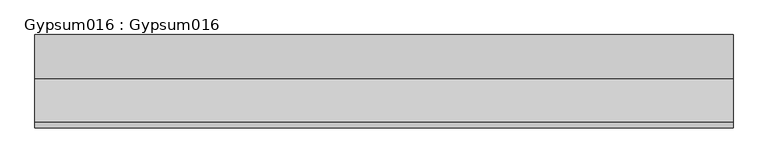
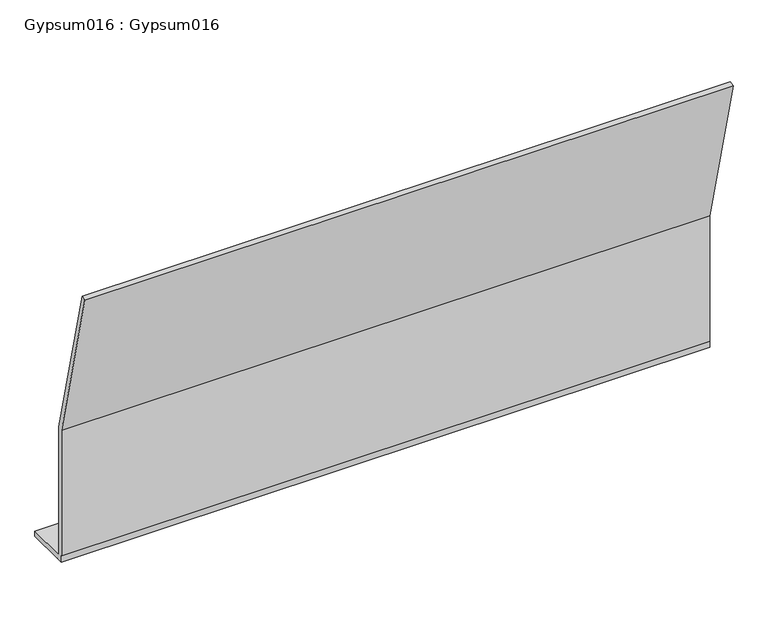
"""IFC4 building model written with IfcOpenShell, lengths in millimetres: proxy geometry, Gypsum016 : Gypsum016."""

from ifc_helpers import new_model, si_unit, frame, origin, place, context, project, spatial, polyline, outline, extrude, source, transform, mapped, element, save


def gypsum016_gypsum016_12ec1e8b(model_context):
    return source(origin(), model_context, "Body", "SweptSolid", [
        extrude(outline(polyline([(10278.0250834, 42906.696), (10404.7574604, 42906.696), (10404.7574604, 42890.821), (10284.5832673, 42890.821), (10284.5832673, 42892.101), (10263.4300834, 42892.101), (10263.4300834, 42913.2541839), (10262.1500834, 42913.2541839), (10262.1500834, 43322.8477886), (10137.3940009, 43821.8721184), (10152.7950131, 43825.7223714), (10278.0250834, 43324.8020904), (10278.0250834, 42906.696)])), frame((3694.2883192, 0.0, 0.0), z_axis=(1.0, 0.0, 0.0), x_axis=(0.0, 1.0, 0.0)), (0.0, 0.0, 1.0), 2000.0),
    ])


if __name__ == "__main__":
    model = new_model("IFC4")
    model_context = context("Model", 3, world=origin())
    ifc_project = project(units=[si_unit("LENGTHUNIT", "METRE", prefix="MILLI")], contexts=[model_context])
    site = spatial("IfcSite", under=ifc_project)
    building = spatial("IfcBuilding", under=site)
    placement = place(None, origin())
    gypsum016_gypsum016_shape = gypsum016_gypsum016_12ec1e8b(model_context)
    element("IfcBuildingElementProxy", 1, Name="Gypsum016 : Gypsum016", ObjectType="Gypsum016 : Gypsum016", at=placement, inside=building, context=model_context, shape_type="MappedRepresentation", body=[
        mapped(gypsum016_gypsum016_shape, transform((0.0, 0.0, 0.0), x_axis=(1.0, 0.0, 0.0), y_axis=(0.0, 1.0, 0.0), z_axis=(0.0, 0.0, 1.0))),
    ])
    save(model, "model.ifc")

# Revit data of these elements
# Type "Gypsum016 : Gypsum016"
#   NameOverride = "Gypsum016"
# Element 1 (IfcBuildingElementProxy, "Gypsum016 : Gypsum016")
#   Materials on its faces: "5/8\" GYPSUM BOARD"
# Materials
#   "5/8\" GYPSUM BOARD": class "Unassigned", colour RGB 214 214 214, transparency 0, Cost = 0
